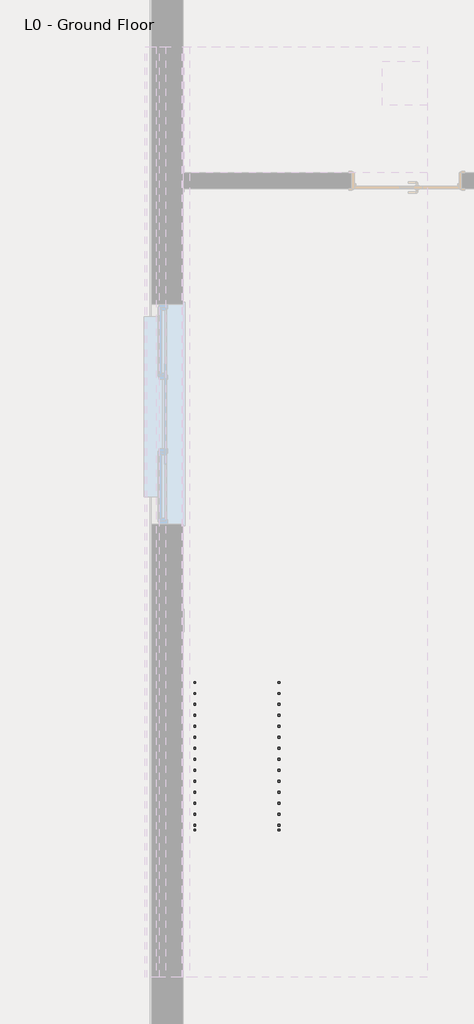
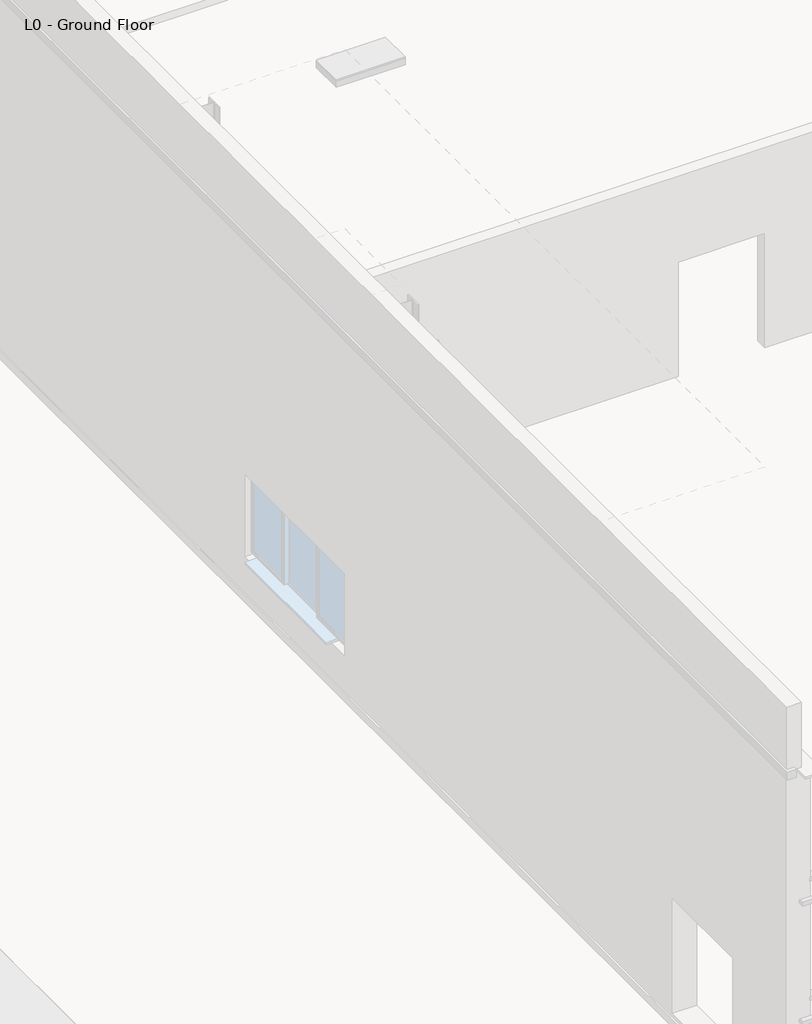
# One storey, part 8 of 14: 2 railings.
"""IFC4 building model written with IfcOpenShell, lengths in millimetres."""

import ifcopenshell
import ifcopenshell.guid

model = None  # the IFC model being written
_history = None  # IfcOwnerHistory: only IFC2X3 demands one
_inside = {}  # id of a spatial element -> (the spatial element, [elements in it])
_under = {}  # id of a project, library or spatial element -> (it, [spatial elements below it])
_declared = {}  # id of a project -> (the project, [libraries it declares])
_typed = {}  # id of a type object -> (the type object, [elements of that type])
_made_of = {}  # id of a material, layer set ... -> (it, [elements and type objects made of it])


def new_model(schema):
    """Start an empty IFC model of exactly this schema.

    Asked for "IFC4X3", IfcOpenShell would pick the latest addendum, in which some entities
    have other attributes; the version numbers below select the first issue.
    IFC2X3 requires an IfcOwnerHistory on every rooted entity: one is made here for all.
    """
    global model, _history
    if schema == "IFC4X3":
        model = ifcopenshell.file(schema_version=(4, 3, 0, 0))
    else:
        model = ifcopenshell.file(schema=schema)
    _inside.clear()
    _under.clear()
    _declared.clear()
    _typed.clear()
    _made_of.clear()
    _history = None
    if model.schema == "IFC2X3":
        org = make("IfcOrganization", Name="unknown")
        user = make(
            "IfcPersonAndOrganization",
            ThePerson=make("IfcPerson", FamilyName="unknown"),
            TheOrganization=org,
        )
        app = make(
            "IfcApplication",
            ApplicationDeveloper=org,
            Version="unknown",
            ApplicationFullName="unknown",
            ApplicationIdentifier="unknown",
        )
        _history = make(
            "IfcOwnerHistory",
            OwningUser=user,
            OwningApplication=app,
            ChangeAction="ADDED",
            CreationDate=0,
        )
    return model


def make(cls, **values):
    """One entity of the class cls with the attributes given. An attribute that is None is left unset."""
    return model.create_entity(
        cls, **{name: value for name, value in values.items() if value is not None}
    )


def rooted(cls, **values):
    """An entity with a GlobalId (a new one), such as an element, a storey or a relation."""
    return make(cls, GlobalId=ifcopenshell.guid.new(), OwnerHistory=_history, **values)


def si_unit(unit_type, name, prefix=None):
    """IfcSIUnit, for example si_unit("LENGTHUNIT", "METRE", prefix="MILLI")."""
    return make("IfcSIUnit", UnitType=unit_type, Prefix=prefix, Name=name)


def assignment(units):
    """IfcUnitAssignment: the units of a project."""
    return None if units is None else make("IfcUnitAssignment", Units=units)


def point(xyz):
    """IfcCartesianPoint."""
    return None if xyz is None else make("IfcCartesianPoint", Coordinates=xyz)


def direction(xyz):
    """IfcDirection."""
    return None if xyz is None else make("IfcDirection", DirectionRatios=xyz)


def frame(location, z_axis=None, x_axis=None):
    """IfcAxis2Placement3D, a coordinate frame: its origin and axes. An axis left out is left unset."""
    return make(
        "IfcAxis2Placement3D",
        Location=point(location),
        Axis=direction(z_axis),
        RefDirection=direction(x_axis),
    )


def origin():
    """The frame at (0, 0, 0) with its axes left unset."""
    return frame((0.0, 0.0, 0.0))


def place(relative_to, where):
    """IfcLocalPlacement: puts the frame where relative to a parent placement (None: the world)."""
    return make(
        "IfcLocalPlacement", PlacementRelTo=relative_to, RelativePlacement=where
    )


def context(
    kind, dimensions, precision=None, world=None, true_north=None, identifier=None
):
    """IfcGeometricRepresentationContext, for example the 3D "Model" context."""
    return make(
        "IfcGeometricRepresentationContext",
        ContextIdentifier=identifier,
        ContextType=kind,
        CoordinateSpaceDimension=dimensions,
        Precision=precision,
        WorldCoordinateSystem=world,
        TrueNorth=true_north,
    )


def project(units=None, contexts=None):
    """IfcProject with its units and contexts."""
    return rooted(
        "IfcProject",
        Name="project",
        RepresentationContexts=contexts,
        UnitsInContext=assignment(units),
    )


def spatial(cls, under=None, at=None, **own):
    """A site, building, storey or space (cls), placed at a placement, below another one or the project."""
    s = rooted(cls, ObjectPlacement=at, **own)
    if under is not None:
        _under.setdefault(under.id(), (under, []))[1].append(s)
    return s


def polyline(points):
    """IfcPolyline through the points."""
    return make("IfcPolyline", Points=[point(p) for p in points])


def outline(outer, holes=None, kind="AREA"):
    """IfcArbitraryClosedProfileDef: a profile drawn as a closed curve; with holes, ...WithVoids."""
    if holes is None:
        return make("IfcArbitraryClosedProfileDef", ProfileType=kind, OuterCurve=outer)
    return make(
        "IfcArbitraryProfileDefWithVoids",
        ProfileType=kind,
        OuterCurve=outer,
        InnerCurves=holes,
    )


def extrude(swept, where, along, depth):
    """IfcExtrudedAreaSolid: the profile swept, set in the frame where, extruded along a direction by depth."""
    return make(
        "IfcExtrudedAreaSolid",
        SweptArea=swept,
        Position=where,
        ExtrudedDirection=direction(along),
        Depth=depth,
    )


def faces_of(points, faces, orient=None, outer=None):
    """IfcFace entities. A face is a list of loops; a loop is a list of indices into points, from 0.

    orient and outer hold one flag for each loop. By default every Orientation is true, the
    first loop of a face is its IfcFaceOuterBound and the others are IfcFaceBound.
    """
    made = []
    for i, loops in enumerate(faces):
        bounds = []
        for j, loop in enumerate(loops):
            is_outer = j == 0 if outer is None else outer[i][j]
            bounds.append(
                make(
                    "IfcFaceOuterBound" if is_outer else "IfcFaceBound",
                    Bound=make("IfcPolyLoop", Polygon=[points[k] for k in loop]),
                    Orientation=True if orient is None else orient[i][j],
                )
            )
        made.append(make("IfcFace", Bounds=bounds))
    return made


def faceted_brep(points, faces, orient=None, outer=None, voids=None):
    """IfcFacetedBrep: a solid bounded by flat faces; with voids (closed shells), ...WithVoids."""
    shared = [point(p) for p in points]
    hull = make("IfcClosedShell", CfsFaces=faces_of(shared, faces, orient, outer))
    if voids is None:
        return make("IfcFacetedBrep", Outer=hull)
    return make(
        "IfcFacetedBrepWithVoids",
        Outer=hull,
        Voids=[
            make(cls, CfsFaces=faces_of(shared, fs, o, b)) for cls, fs, o, b in voids
        ],
    )


def shape(context_of_items, identifier, shape_type, items):
    """IfcShapeRepresentation: the items that make up one representation, for example the "Body"."""
    return make(
        "IfcShapeRepresentation",
        ContextOfItems=context_of_items,
        RepresentationIdentifier=identifier,
        RepresentationType=shape_type,
        Items=items,
    )


def made_of(thing, what):
    """Note that an element or type object is made of a material, layer set ...; save() writes the relation."""
    if what is not None:
        _made_of.setdefault(what.id(), (what, []))[1].append(thing)
    return thing


def element(
    cls,
    number,
    at=None,
    inside=None,
    cuts=None,
    type_object=None,
    material=None,
    context=None,
    identifier="Body",
    shape_type=None,
    held_by="IfcProductDefinitionShape",
    body=None,
    shapes=None,
    **own,
):
    """One element of the class cls, such as IfcWall. Its Tag is "e" and its number.

    at: its placement. inside: the storey or other place that contains it. cuts: it is an
    opening in that element (IfcRelVoidsElement). A single representation is given by context,
    identifier, shape_type and body (its items); several are given by shapes. held_by: the class
    of the entity that holds the representations. save() writes the other relations.
    """
    e = rooted(cls, Tag="e%d" % number, ObjectPlacement=at, **own)
    if body is not None:
        shapes = [shape(context, identifier, shape_type, body)]
    if shapes is not None:
        e.Representation = make(held_by, Representations=shapes)
    if inside is not None:
        _inside.setdefault(inside.id(), (inside, []))[1].append(e)
    if cuts is not None:
        rooted(
            "IfcRelVoidsElement", RelatingBuildingElement=cuts, RelatedOpeningElement=e
        )
    if type_object is not None:
        _typed.setdefault(type_object.id(), (type_object, []))[1].append(e)
    return made_of(e, material)


def aggregate(whole, parts):
    """IfcRelAggregates: a whole, such as a stair, and the parts it consists of."""
    return rooted("IfcRelAggregates", RelatingObject=whole, RelatedObjects=parts)


def save(model, path):
    """Write the relations noted so far, then the file.

    IfcRelAggregates (storeys below a building ...), IfcRelContainedInSpatialStructure (elements
    in a storey), IfcRelDefinesByType, IfcRelAssociatesMaterial and IfcRelDeclares: one each for
    every whole, place, type object, material and project.
    """
    for whole, parts in _under.values():
        aggregate(whole, parts)
    for where, things in _inside.values():
        rooted(
            "IfcRelContainedInSpatialStructure",
            RelatedElements=things,
            RelatingStructure=where,
        )
    for kind, things in _typed.values():
        rooted("IfcRelDefinesByType", RelatedObjects=things, RelatingType=kind)
    for what, things in _made_of.values():
        rooted("IfcRelAssociatesMaterial", RelatedObjects=things, RelatingMaterial=what)
    for by, libraries in _declared.values():
        rooted("IfcRelDeclares", RelatingContext=by, RelatedDefinitions=libraries)
    model.write(path)


model = new_model("IFC4")

# Units and contexts
model_context = context("Model", 3, world=origin())
ifc_project = project(units=[si_unit("LENGTHUNIT", "METRE", prefix="MILLI")], contexts=[model_context])

# Site, building, storey
site = spatial("IfcSite", under=ifc_project)
building = spatial("IfcBuilding", under=site)
storey = spatial("IfcBuildingStorey", under=building, Name="L0 - Ground Floor", Elevation=0.0)

# Railings
placement = place(None, origin())
element("IfcRailing", 1, ObjectType="1100mm", at=placement, inside=storey, context=model_context, shape_type="SolidModel", body=[
    faceted_brep([(-5716.2916692, -13929.5546689, 1266.6666667), (-5716.2916692, -13929.5546689, 1209.4687214), (-5666.2916692, -13929.5546689, 1209.4687214), (-5666.2916692, -13929.5546689, 1266.6666667), (-5716.2916692, -11829.5546689, 2433.3333333), (-5716.2916692, -11816.5983675, 2383.3333333), (-5666.2916692, -11816.5983675, 2383.3333333), (-5666.2916692, -11829.5546689, 2433.3333333), (-5716.2916692, -10929.5546689, 2433.3333333), (-5716.2916692, -10916.5983675, 2383.3333333), (-5666.2916692, -10916.5983675, 2383.3333333), (-5666.2916692, -10929.5546689, 2433.3333333), (-5716.2916692, -8529.5546689, 3766.6666667), (-5716.2916692, -8516.5983675, 3716.6666667), (-5666.2916692, -8516.5983675, 3716.6666667), (-5666.2916692, -8529.5546689, 3766.6666667), (-5716.2916692, -7629.5546689, 3766.6666667), (-5716.2916692, -7616.5983675, 3716.6666667), (-5666.2916692, -7616.5983675, 3716.6666667), (-5666.2916692, -7629.5546689, 3766.6666667), (-5716.2916692, -5229.5546689, 5100.0), (-5666.2916692, -5229.5546689, 5100.0), (-5666.2916692, -5229.5546689, 5042.8020548), (-5716.2916692, -5229.5546689, 5042.8020548)], [[[0, 1, 2, 3]], [[1, 0, 4, 5]], [[2, 1, 5, 6]], [[3, 2, 6, 7]], [[0, 3, 7, 4]], [[5, 4, 8, 9]], [[6, 5, 9, 10]], [[7, 6, 10, 11]], [[4, 7, 11, 8]], [[9, 8, 12, 13]], [[10, 9, 13, 14]], [[11, 10, 14, 15]], [[8, 11, 15, 12]], [[13, 12, 16, 17]], [[14, 13, 17, 18]], [[15, 14, 18, 19]], [[12, 15, 19, 16]], [[20, 21, 22, 23]], [[17, 16, 20, 23]], [[18, 17, 23, 22]], [[19, 18, 22, 21]], [[16, 19, 21, 20]]]),
    extrude(outline(polyline([(-5317.0546689, 3833.3333333), (-5317.0546689, 4994.1909437), (-5292.0546689, 5008.0798326), (-5292.0546689, 3833.3333333), (-5317.0546689, 3833.3333333)])), frame((-5703.7916692, 0.0, 0.0), z_axis=(1.0, 0.0, 0.0), x_axis=(0.0, 1.0, 0.0)), (0.0, 0.0, 1.0), 25.0),
    extrude(outline(polyline([(-5467.0546689, 3833.3333333), (-5467.0546689, 4910.8576103), (-5442.0546689, 4924.7464992), (-5442.0546689, 3833.3333333), (-5467.0546689, 3833.3333333)])), frame((-5703.7916692, 0.0, 0.0), z_axis=(1.0, 0.0, 0.0), x_axis=(0.0, 1.0, 0.0)), (0.0, 0.0, 1.0), 25.0),
    extrude(outline(polyline([(-5617.0546689, 3666.6666667), (-5617.0546689, 4827.524277), (-5592.0546689, 4841.4131659), (-5592.0546689, 3666.6666667), (-5617.0546689, 3666.6666667)])), frame((-5703.7916692, 0.0, 0.0), z_axis=(1.0, 0.0, 0.0), x_axis=(0.0, 1.0, 0.0)), (0.0, 0.0, 1.0), 25.0),
    extrude(outline(polyline([(-5767.0546689, 3666.6666667), (-5767.0546689, 4744.1909437), (-5742.0546689, 4758.0798326), (-5742.0546689, 3666.6666667), (-5767.0546689, 3666.6666667)])), frame((-5703.7916692, 0.0, 0.0), z_axis=(1.0, 0.0, 0.0), x_axis=(0.0, 1.0, 0.0)), (0.0, 0.0, 1.0), 25.0),
    extrude(outline(polyline([(-5917.0546689, 3500.0), (-5917.0546689, 4660.8576103), (-5892.0546689, 4674.7464992), (-5892.0546689, 3500.0), (-5917.0546689, 3500.0)])), frame((-5703.7916692, 0.0, 0.0), z_axis=(1.0, 0.0, 0.0), x_axis=(0.0, 1.0, 0.0)), (0.0, 0.0, 1.0), 25.0),
    extrude(outline(polyline([(-6067.0546689, 3500.0), (-6067.0546689, 4577.524277), (-6042.0546689, 4591.4131659), (-6042.0546689, 3500.0), (-6067.0546689, 3500.0)])), frame((-5703.7916692, 0.0, 0.0), z_axis=(1.0, 0.0, 0.0), x_axis=(0.0, 1.0, 0.0)), (0.0, 0.0, 1.0), 25.0),
    extrude(outline(polyline([(-6217.0546689, 3333.3333333), (-6217.0546689, 4494.1909437), (-6192.0546689, 4508.0798326), (-6192.0546689, 3333.3333333), (-6217.0546689, 3333.3333333)])), frame((-5703.7916692, 0.0, 0.0), z_axis=(1.0, 0.0, 0.0), x_axis=(0.0, 1.0, 0.0)), (0.0, 0.0, 1.0), 25.0),
    extrude(outline(polyline([(-6367.0546689, 3333.3333333), (-6367.0546689, 4410.8576103), (-6342.0546689, 4424.7464992), (-6342.0546689, 3333.3333333), (-6367.0546689, 3333.3333333)])), frame((-5703.7916692, 0.0, 0.0), z_axis=(1.0, 0.0, 0.0), x_axis=(0.0, 1.0, 0.0)), (0.0, 0.0, 1.0), 25.0),
    extrude(outline(polyline([(-6517.0546689, 3166.6666667), (-6517.0546689, 4327.524277), (-6492.0546689, 4341.4131659), (-6492.0546689, 3166.6666667), (-6517.0546689, 3166.6666667)])), frame((-5703.7916692, 0.0, 0.0), z_axis=(1.0, 0.0, 0.0), x_axis=(0.0, 1.0, 0.0)), (0.0, 0.0, 1.0), 25.0),
    extrude(outline(polyline([(-6667.0546689, 3166.6666667), (-6667.0546689, 4244.1909437), (-6642.0546689, 4258.0798326), (-6642.0546689, 3166.6666667), (-6667.0546689, 3166.6666667)])), frame((-5703.7916692, 0.0, 0.0), z_axis=(1.0, 0.0, 0.0), x_axis=(0.0, 1.0, 0.0)), (0.0, 0.0, 1.0), 25.0),
    extrude(outline(polyline([(-6817.0546689, 3000.0), (-6817.0546689, 4160.8576103), (-6792.0546689, 4174.7464992), (-6792.0546689, 3000.0), (-6817.0546689, 3000.0)])), frame((-5703.7916692, 0.0, 0.0), z_axis=(1.0, 0.0, 0.0), x_axis=(0.0, 1.0, 0.0)), (0.0, 0.0, 1.0), 25.0),
    extrude(outline(polyline([(-6967.0546689, 3000.0), (-6967.0546689, 4077.524277), (-6942.0546689, 4091.4131659), (-6942.0546689, 3000.0), (-6967.0546689, 3000.0)])), frame((-5703.7916692, 0.0, 0.0), z_axis=(1.0, 0.0, 0.0), x_axis=(0.0, 1.0, 0.0)), (0.0, 0.0, 1.0), 25.0),
    extrude(outline(polyline([(-7117.0546689, 2833.3333333), (-7117.0546689, 3994.1909437), (-7092.0546689, 4008.0798326), (-7092.0546689, 2833.3333333), (-7117.0546689, 2833.3333333)])), frame((-5703.7916692, 0.0, 0.0), z_axis=(1.0, 0.0, 0.0), x_axis=(0.0, 1.0, 0.0)), (0.0, 0.0, 1.0), 25.0),
    extrude(outline(polyline([(-7267.0546689, 2833.3333333), (-7267.0546689, 3910.8576103), (-7242.0546689, 3924.7464992), (-7242.0546689, 2833.3333333), (-7267.0546689, 2833.3333333)])), frame((-5703.7916692, 0.0, 0.0), z_axis=(1.0, 0.0, 0.0), x_axis=(0.0, 1.0, 0.0)), (0.0, 0.0, 1.0), 25.0),
    extrude(outline(polyline([(-7417.0546689, 2666.6666667), (-7417.0546689, 3827.524277), (-7392.0546689, 3841.4131659), (-7392.0546689, 2666.6666667), (-7417.0546689, 2666.6666667)])), frame((-5703.7916692, 0.0, 0.0), z_axis=(1.0, 0.0, 0.0), x_axis=(0.0, 1.0, 0.0)), (0.0, 0.0, 1.0), 25.0),
    extrude(outline(polyline([(-7567.0546689, 2666.6666667), (-7567.0546689, 3744.1909437), (-7542.0546689, 3758.0798326), (-7542.0546689, 2666.6666667), (-7567.0546689, 2666.6666667)])), frame((-5703.7916692, 0.0, 0.0), z_axis=(1.0, 0.0, 0.0), x_axis=(0.0, 1.0, 0.0)), (0.0, 0.0, 1.0), 25.0),
    extrude(outline(polyline([(-5678.7916692, -7717.0546689), (-5703.7916692, -7717.0546689), (-5703.7916692, -7692.0546689), (-5678.7916692, -7692.0546689), (-5678.7916692, -7717.0546689)])), frame((0.0, 0.0, 2666.6666667), z_axis=(0.0, 0.0, 1.0), x_axis=(1.0, 0.0, 0.0)), (0.0, 0.0, 1.0), 1050.0),
    extrude(outline(polyline([(-5678.7916692, -7867.0546689), (-5703.7916692, -7867.0546689), (-5703.7916692, -7842.0546689), (-5678.7916692, -7842.0546689), (-5678.7916692, -7867.0546689)])), frame((0.0, 0.0, 2666.6666667), z_axis=(0.0, 0.0, 1.0), x_axis=(1.0, 0.0, 0.0)), (0.0, 0.0, 1.0), 1050.0),
    extrude(outline(polyline([(-5678.7916692, -8017.0546689), (-5703.7916692, -8017.0546689), (-5703.7916692, -7992.0546689), (-5678.7916692, -7992.0546689), (-5678.7916692, -8017.0546689)])), frame((0.0, 0.0, 2666.6666667), z_axis=(0.0, 0.0, 1.0), x_axis=(1.0, 0.0, 0.0)), (0.0, 0.0, 1.0), 1050.0),
    extrude(outline(polyline([(-5678.7916692, -8167.0546689), (-5703.7916692, -8167.0546689), (-5703.7916692, -8142.0546689), (-5678.7916692, -8142.0546689), (-5678.7916692, -8167.0546689)])), frame((0.0, 0.0, 2666.6666667), z_axis=(0.0, 0.0, 1.0), x_axis=(1.0, 0.0, 0.0)), (0.0, 0.0, 1.0), 1050.0),
    extrude(outline(polyline([(-5678.7916692, -8317.0546689), (-5703.7916692, -8317.0546689), (-5703.7916692, -8292.0546689), (-5678.7916692, -8292.0546689), (-5678.7916692, -8317.0546689)])), frame((0.0, 0.0, 2666.6666667), z_axis=(0.0, 0.0, 1.0), x_axis=(1.0, 0.0, 0.0)), (0.0, 0.0, 1.0), 1050.0),
    extrude(outline(polyline([(-5678.7916692, -8467.0546689), (-5703.7916692, -8467.0546689), (-5703.7916692, -8442.0546689), (-5678.7916692, -8442.0546689), (-5678.7916692, -8467.0546689)])), frame((0.0, 0.0, 2666.6666667), z_axis=(0.0, 0.0, 1.0), x_axis=(1.0, 0.0, 0.0)), (0.0, 0.0, 1.0), 1050.0),
    extrude(outline(polyline([(-8617.0546689, 2500.0), (-8617.0546689, 3660.8576103), (-8592.0546689, 3674.7464992), (-8592.0546689, 2500.0), (-8617.0546689, 2500.0)])), frame((-5703.7916692, 0.0, 0.0), z_axis=(1.0, 0.0, 0.0), x_axis=(0.0, 1.0, 0.0)), (0.0, 0.0, 1.0), 25.0),
    extrude(outline(polyline([(-8767.0546689, 2500.0), (-8767.0546689, 3577.524277), (-8742.0546689, 3591.4131659), (-8742.0546689, 2500.0), (-8767.0546689, 2500.0)])), frame((-5703.7916692, 0.0, 0.0), z_axis=(1.0, 0.0, 0.0), x_axis=(0.0, 1.0, 0.0)), (0.0, 0.0, 1.0), 25.0),
    extrude(outline(polyline([(-8917.0546689, 2333.3333333), (-8917.0546689, 3494.1909437), (-8892.0546689, 3508.0798326), (-8892.0546689, 2333.3333333), (-8917.0546689, 2333.3333333)])), frame((-5703.7916692, 0.0, 0.0), z_axis=(1.0, 0.0, 0.0), x_axis=(0.0, 1.0, 0.0)), (0.0, 0.0, 1.0), 25.0),
    extrude(outline(polyline([(-9067.0546689, 2333.3333333), (-9067.0546689, 3410.8576103), (-9042.0546689, 3424.7464992), (-9042.0546689, 2333.3333333), (-9067.0546689, 2333.3333333)])), frame((-5703.7916692, 0.0, 0.0), z_axis=(1.0, 0.0, 0.0), x_axis=(0.0, 1.0, 0.0)), (0.0, 0.0, 1.0), 25.0),
    extrude(outline(polyline([(-9217.0546689, 2166.6666667), (-9217.0546689, 3327.524277), (-9192.0546689, 3341.4131659), (-9192.0546689, 2166.6666667), (-9217.0546689, 2166.6666667)])), frame((-5703.7916692, 0.0, 0.0), z_axis=(1.0, 0.0, 0.0), x_axis=(0.0, 1.0, 0.0)), (0.0, 0.0, 1.0), 25.0),
    extrude(outline(polyline([(-9367.0546689, 2166.6666667), (-9367.0546689, 3244.1909437), (-9342.0546689, 3258.0798326), (-9342.0546689, 2166.6666667), (-9367.0546689, 2166.6666667)])), frame((-5703.7916692, 0.0, 0.0), z_axis=(1.0, 0.0, 0.0), x_axis=(0.0, 1.0, 0.0)), (0.0, 0.0, 1.0), 25.0),
    extrude(outline(polyline([(-9517.0546689, 2000.0), (-9517.0546689, 3160.8576103), (-9492.0546689, 3174.7464992), (-9492.0546689, 2000.0), (-9517.0546689, 2000.0)])), frame((-5703.7916692, 0.0, 0.0), z_axis=(1.0, 0.0, 0.0), x_axis=(0.0, 1.0, 0.0)), (0.0, 0.0, 1.0), 25.0),
    extrude(outline(polyline([(-9667.0546689, 2000.0), (-9667.0546689, 3077.524277), (-9642.0546689, 3091.4131659), (-9642.0546689, 2000.0), (-9667.0546689, 2000.0)])), frame((-5703.7916692, 0.0, 0.0), z_axis=(1.0, 0.0, 0.0), x_axis=(0.0, 1.0, 0.0)), (0.0, 0.0, 1.0), 25.0),
    extrude(outline(polyline([(-9817.0546689, 1833.3333333), (-9817.0546689, 2994.1909437), (-9792.0546689, 3008.0798326), (-9792.0546689, 1833.3333333), (-9817.0546689, 1833.3333333)])), frame((-5703.7916692, 0.0, 0.0), z_axis=(1.0, 0.0, 0.0), x_axis=(0.0, 1.0, 0.0)), (0.0, 0.0, 1.0), 25.0),
    extrude(outline(polyline([(-9967.0546689, 1833.3333333), (-9967.0546689, 2910.8576103), (-9942.0546689, 2924.7464992), (-9942.0546689, 1833.3333333), (-9967.0546689, 1833.3333333)])), frame((-5703.7916692, 0.0, 0.0), z_axis=(1.0, 0.0, 0.0), x_axis=(0.0, 1.0, 0.0)), (0.0, 0.0, 1.0), 25.0),
    extrude(outline(polyline([(-10117.0546689, 1666.6666667), (-10117.0546689, 2827.524277), (-10092.0546689, 2841.4131659), (-10092.0546689, 1666.6666667), (-10117.0546689, 1666.6666667)])), frame((-5703.7916692, 0.0, 0.0), z_axis=(1.0, 0.0, 0.0), x_axis=(0.0, 1.0, 0.0)), (0.0, 0.0, 1.0), 25.0),
    extrude(outline(polyline([(-10267.0546689, 1666.6666667), (-10267.0546689, 2744.1909437), (-10242.0546689, 2758.0798326), (-10242.0546689, 1666.6666667), (-10267.0546689, 1666.6666667)])), frame((-5703.7916692, 0.0, 0.0), z_axis=(1.0, 0.0, 0.0), x_axis=(0.0, 1.0, 0.0)), (0.0, 0.0, 1.0), 25.0),
    extrude(outline(polyline([(-10417.0546689, 1500.0), (-10417.0546689, 2660.8576103), (-10392.0546689, 2674.7464992), (-10392.0546689, 1500.0), (-10417.0546689, 1500.0)])), frame((-5703.7916692, 0.0, 0.0), z_axis=(1.0, 0.0, 0.0), x_axis=(0.0, 1.0, 0.0)), (0.0, 0.0, 1.0), 25.0),
    extrude(outline(polyline([(-10567.0546689, 1500.0), (-10567.0546689, 2577.524277), (-10542.0546689, 2591.4131659), (-10542.0546689, 1500.0), (-10567.0546689, 1500.0)])), frame((-5703.7916692, 0.0, 0.0), z_axis=(1.0, 0.0, 0.0), x_axis=(0.0, 1.0, 0.0)), (0.0, 0.0, 1.0), 25.0),
    extrude(outline(polyline([(-10717.0546689, 1333.3333333), (-10717.0546689, 2494.1909437), (-10692.0546689, 2508.0798326), (-10692.0546689, 1333.3333333), (-10717.0546689, 1333.3333333)])), frame((-5703.7916692, 0.0, 0.0), z_axis=(1.0, 0.0, 0.0), x_axis=(0.0, 1.0, 0.0)), (0.0, 0.0, 1.0), 25.0),
    extrude(outline(polyline([(-10867.0546689, 1333.3333333), (-10867.0546689, 2410.8576103), (-10842.0546689, 2424.7464992), (-10842.0546689, 1333.3333333), (-10867.0546689, 1333.3333333)])), frame((-5703.7916692, 0.0, 0.0), z_axis=(1.0, 0.0, 0.0), x_axis=(0.0, 1.0, 0.0)), (0.0, 0.0, 1.0), 25.0),
    extrude(outline(polyline([(-5678.7916692, -11017.0546689), (-5703.7916692, -11017.0546689), (-5703.7916692, -10992.0546689), (-5678.7916692, -10992.0546689), (-5678.7916692, -11017.0546689)])), frame((0.0, 0.0, 1333.3333333), z_axis=(0.0, 0.0, 1.0), x_axis=(1.0, 0.0, 0.0)), (0.0, 0.0, 1.0), 1050.0),
    extrude(outline(polyline([(-5678.7916692, -11167.0546689), (-5703.7916692, -11167.0546689), (-5703.7916692, -11142.0546689), (-5678.7916692, -11142.0546689), (-5678.7916692, -11167.0546689)])), frame((0.0, 0.0, 1333.3333333), z_axis=(0.0, 0.0, 1.0), x_axis=(1.0, 0.0, 0.0)), (0.0, 0.0, 1.0), 1050.0),
    extrude(outline(polyline([(-5678.7916692, -11317.0546689), (-5703.7916692, -11317.0546689), (-5703.7916692, -11292.0546689), (-5678.7916692, -11292.0546689), (-5678.7916692, -11317.0546689)])), frame((0.0, 0.0, 1333.3333333), z_axis=(0.0, 0.0, 1.0), x_axis=(1.0, 0.0, 0.0)), (0.0, 0.0, 1.0), 1050.0),
    extrude(outline(polyline([(-5678.7916692, -11467.0546689), (-5703.7916692, -11467.0546689), (-5703.7916692, -11442.0546689), (-5678.7916692, -11442.0546689), (-5678.7916692, -11467.0546689)])), frame((0.0, 0.0, 1333.3333333), z_axis=(0.0, 0.0, 1.0), x_axis=(1.0, 0.0, 0.0)), (0.0, 0.0, 1.0), 1050.0),
    extrude(outline(polyline([(-5678.7916692, -11617.0546689), (-5703.7916692, -11617.0546689), (-5703.7916692, -11592.0546689), (-5678.7916692, -11592.0546689), (-5678.7916692, -11617.0546689)])), frame((0.0, 0.0, 1333.3333333), z_axis=(0.0, 0.0, 1.0), x_axis=(1.0, 0.0, 0.0)), (0.0, 0.0, 1.0), 1050.0),
    extrude(outline(polyline([(-5678.7916692, -11767.0546689), (-5703.7916692, -11767.0546689), (-5703.7916692, -11742.0546689), (-5678.7916692, -11742.0546689), (-5678.7916692, -11767.0546689)])), frame((0.0, 0.0, 1333.3333333), z_axis=(0.0, 0.0, 1.0), x_axis=(1.0, 0.0, 0.0)), (0.0, 0.0, 1.0), 1050.0),
    extrude(outline(polyline([(-11917.0546689, 1166.6666667), (-11917.0546689, 2327.524277), (-11892.0546689, 2341.4131659), (-11892.0546689, 1166.6666667), (-11917.0546689, 1166.6666667)])), frame((-5703.7916692, 0.0, 0.0), z_axis=(1.0, 0.0, 0.0), x_axis=(0.0, 1.0, 0.0)), (0.0, 0.0, 1.0), 25.0),
    extrude(outline(polyline([(-12067.0546689, 1166.6666667), (-12067.0546689, 2244.1909437), (-12042.0546689, 2258.0798326), (-12042.0546689, 1166.6666667), (-12067.0546689, 1166.6666667)])), frame((-5703.7916692, 0.0, 0.0), z_axis=(1.0, 0.0, 0.0), x_axis=(0.0, 1.0, 0.0)), (0.0, 0.0, 1.0), 25.0),
    extrude(outline(polyline([(-12217.0546689, 1000.0), (-12217.0546689, 2160.8576103), (-12192.0546689, 2174.7464992), (-12192.0546689, 1000.0), (-12217.0546689, 1000.0)])), frame((-5703.7916692, 0.0, 0.0), z_axis=(1.0, 0.0, 0.0), x_axis=(0.0, 1.0, 0.0)), (0.0, 0.0, 1.0), 25.0),
    extrude(outline(polyline([(-12367.0546689, 1000.0), (-12367.0546689, 2077.524277), (-12342.0546689, 2091.4131659), (-12342.0546689, 1000.0), (-12367.0546689, 1000.0)])), frame((-5703.7916692, 0.0, 0.0), z_axis=(1.0, 0.0, 0.0), x_axis=(0.0, 1.0, 0.0)), (0.0, 0.0, 1.0), 25.0),
    extrude(outline(polyline([(-12517.0546689, 833.3333333), (-12517.0546689, 1994.1909437), (-12492.0546689, 2008.0798326), (-12492.0546689, 833.3333333), (-12517.0546689, 833.3333333)])), frame((-5703.7916692, 0.0, 0.0), z_axis=(1.0, 0.0, 0.0), x_axis=(0.0, 1.0, 0.0)), (0.0, 0.0, 1.0), 25.0),
    extrude(outline(polyline([(-12667.0546689, 833.3333333), (-12667.0546689, 1910.8576103), (-12642.0546689, 1924.7464992), (-12642.0546689, 833.3333333), (-12667.0546689, 833.3333333)])), frame((-5703.7916692, 0.0, 0.0), z_axis=(1.0, 0.0, 0.0), x_axis=(0.0, 1.0, 0.0)), (0.0, 0.0, 1.0), 25.0),
    extrude(outline(polyline([(-12817.0546689, 666.6666667), (-12817.0546689, 1827.524277), (-12792.0546689, 1841.4131659), (-12792.0546689, 666.6666667), (-12817.0546689, 666.6666667)])), frame((-5703.7916692, 0.0, 0.0), z_axis=(1.0, 0.0, 0.0), x_axis=(0.0, 1.0, 0.0)), (0.0, 0.0, 1.0), 25.0),
    extrude(outline(polyline([(-12967.0546689, 666.6666667), (-12967.0546689, 1744.1909437), (-12942.0546689, 1758.0798326), (-12942.0546689, 666.6666667), (-12967.0546689, 666.6666667)])), frame((-5703.7916692, 0.0, 0.0), z_axis=(1.0, 0.0, 0.0), x_axis=(0.0, 1.0, 0.0)), (0.0, 0.0, 1.0), 25.0),
    extrude(outline(polyline([(-13117.0546689, 500.0), (-13117.0546689, 1660.8576103), (-13092.0546689, 1674.7464992), (-13092.0546689, 500.0), (-13117.0546689, 500.0)])), frame((-5703.7916692, 0.0, 0.0), z_axis=(1.0, 0.0, 0.0), x_axis=(0.0, 1.0, 0.0)), (0.0, 0.0, 1.0), 25.0),
    extrude(outline(polyline([(-13267.0546689, 500.0), (-13267.0546689, 1577.524277), (-13242.0546689, 1591.4131659), (-13242.0546689, 500.0), (-13267.0546689, 500.0)])), frame((-5703.7916692, 0.0, 0.0), z_axis=(1.0, 0.0, 0.0), x_axis=(0.0, 1.0, 0.0)), (0.0, 0.0, 1.0), 25.0),
    extrude(outline(polyline([(-13417.0546689, 333.3333333), (-13417.0546689, 1494.1909437), (-13392.0546689, 1508.0798326), (-13392.0546689, 333.3333333), (-13417.0546689, 333.3333333)])), frame((-5703.7916692, 0.0, 0.0), z_axis=(1.0, 0.0, 0.0), x_axis=(0.0, 1.0, 0.0)), (0.0, 0.0, 1.0), 25.0),
    extrude(outline(polyline([(-13567.0546689, 333.3333333), (-13567.0546689, 1410.8576103), (-13542.0546689, 1424.7464992), (-13542.0546689, 333.3333333), (-13567.0546689, 333.3333333)])), frame((-5703.7916692, 0.0, 0.0), z_axis=(1.0, 0.0, 0.0), x_axis=(0.0, 1.0, 0.0)), (0.0, 0.0, 1.0), 25.0),
    extrude(outline(polyline([(-13717.0546689, 166.6666667), (-13717.0546689, 1327.524277), (-13692.0546689, 1341.4131659), (-13692.0546689, 166.6666667), (-13717.0546689, 166.6666667)])), frame((-5703.7916692, 0.0, 0.0), z_axis=(1.0, 0.0, 0.0), x_axis=(0.0, 1.0, 0.0)), (0.0, 0.0, 1.0), 25.0),
    extrude(outline(polyline([(-13867.0546689, 166.6666667), (-13867.0546689, 1244.1909437), (-13842.0546689, 1258.0798326), (-13842.0546689, 166.6666667), (-13867.0546689, 166.6666667)])), frame((-5703.7916692, 0.0, 0.0), z_axis=(1.0, 0.0, 0.0), x_axis=(0.0, 1.0, 0.0)), (0.0, 0.0, 1.0), 25.0),
    extrude(outline(polyline([(-5678.7916692, -7642.0546689), (-5703.7916692, -7642.0546689), (-5703.7916692, -7617.0546689), (-5678.7916692, -7617.0546689), (-5678.7916692, -7642.0546689)])), frame((0.0, 0.0, 2666.6666667), z_axis=(0.0, 0.0, 1.0), x_axis=(1.0, 0.0, 0.0)), (0.0, 0.0, 1.0), 1050.0),
    extrude(outline(polyline([(-8542.0546689, 2666.6666667), (-8542.0546689, 3702.524277), (-8517.0546689, 3716.4131659), (-8517.0546689, 2666.6666667), (-8542.0546689, 2666.6666667)])), frame((-5703.7916692, 0.0, 0.0), z_axis=(1.0, 0.0, 0.0), x_axis=(0.0, 1.0, 0.0)), (0.0, 0.0, 1.0), 25.0),
    extrude(outline(polyline([(-5678.7916692, -10942.0546689), (-5703.7916692, -10942.0546689), (-5703.7916692, -10917.0546689), (-5678.7916692, -10917.0546689), (-5678.7916692, -10942.0546689)])), frame((0.0, 0.0, 1333.3333333), z_axis=(0.0, 0.0, 1.0), x_axis=(1.0, 0.0, 0.0)), (0.0, 0.0, 1.0), 1050.0),
    extrude(outline(polyline([(-11842.0546689, 1333.3333333), (-11842.0546689, 2369.1909437), (-11817.0546689, 2383.0798326), (-11817.0546689, 1333.3333333), (-11842.0546689, 1333.3333333)])), frame((-5703.7916692, 0.0, 0.0), z_axis=(1.0, 0.0, 0.0), x_axis=(0.0, 1.0, 0.0)), (0.0, 0.0, 1.0), 25.0),
    extrude(outline(polyline([(-5254.5546689, 3833.3333333), (-5254.5546689, 5028.9131659), (-5229.5546689, 5042.8020548), (-5229.5546689, 3833.3333333), (-5254.5546689, 3833.3333333)])), frame((-5703.7916692, 0.0, 0.0), z_axis=(1.0, 0.0, 0.0), x_axis=(0.0, 1.0, 0.0)), (0.0, 0.0, 1.0), 25.0),
    extrude(outline(polyline([(-13929.5546689, 166.6666667), (-13929.5546689, 1209.4687214), (-13904.5546689, 1223.3576103), (-13904.5546689, 166.6666667), (-13929.5546689, 166.6666667)])), frame((-5703.7916692, 0.0, 0.0), z_axis=(1.0, 0.0, 0.0), x_axis=(0.0, 1.0, 0.0)), (0.0, 0.0, 1.0), 25.0),
])
element("IfcRailing", 2, ObjectType="1100mm", at=placement, inside=storey, context=model_context, shape_type="SolidModel", body=[
    faceted_brep([(-6865.4916692, -13929.5546689, 1266.6666667), (-6865.4916692, -13929.5546689, 1209.4687214), (-6815.4916692, -13929.5546689, 1209.4687214), (-6815.4916692, -13929.5546689, 1266.6666667), (-6865.4916692, -11829.5546689, 2433.3333333), (-6865.4916692, -11816.5983675, 2383.3333333), (-6815.4916692, -11816.5983675, 2383.3333333), (-6815.4916692, -11829.5546689, 2433.3333333), (-6865.4916692, -10929.5546689, 2433.3333333), (-6865.4916692, -10916.5983675, 2383.3333333), (-6815.4916692, -10916.5983675, 2383.3333333), (-6815.4916692, -10929.5546689, 2433.3333333), (-6865.4916692, -8529.5546689, 3766.6666667), (-6865.4916692, -8516.5983675, 3716.6666667), (-6815.4916692, -8516.5983675, 3716.6666667), (-6815.4916692, -8529.5546689, 3766.6666667), (-6865.4916692, -7629.5546689, 3766.6666667), (-6865.4916692, -7616.5983675, 3716.6666667), (-6815.4916692, -7616.5983675, 3716.6666667), (-6815.4916692, -7629.5546689, 3766.6666667), (-6865.4916692, -5229.5546689, 5100.0), (-6815.4916692, -5229.5546689, 5100.0), (-6815.4916692, -5229.5546689, 5042.8020548), (-6865.4916692, -5229.5546689, 5042.8020548)], [[[0, 1, 2, 3]], [[1, 0, 4, 5]], [[2, 1, 5, 6]], [[3, 2, 6, 7]], [[0, 3, 7, 4]], [[5, 4, 8, 9]], [[6, 5, 9, 10]], [[7, 6, 10, 11]], [[4, 7, 11, 8]], [[9, 8, 12, 13]], [[10, 9, 13, 14]], [[11, 10, 14, 15]], [[8, 11, 15, 12]], [[13, 12, 16, 17]], [[14, 13, 17, 18]], [[15, 14, 18, 19]], [[12, 15, 19, 16]], [[20, 21, 22, 23]], [[17, 16, 20, 23]], [[18, 17, 23, 22]], [[19, 18, 22, 21]], [[16, 19, 21, 20]]]),
    extrude(outline(polyline([(-5317.0546689, 4994.1909437), (-5292.0546689, 5008.0798326), (-5292.0546689, 3833.3333333), (-5317.0546689, 3833.3333333), (-5317.0546689, 4994.1909437)])), frame((-6852.9916692, 0.0, 0.0), z_axis=(1.0, 0.0, 0.0), x_axis=(0.0, 1.0, 0.0)), (0.0, 0.0, 1.0), 25.0),
    extrude(outline(polyline([(-5467.0546689, 4910.8576103), (-5442.0546689, 4924.7464992), (-5442.0546689, 3833.3333333), (-5467.0546689, 3833.3333333), (-5467.0546689, 4910.8576103)])), frame((-6852.9916692, 0.0, 0.0), z_axis=(1.0, 0.0, 0.0), x_axis=(0.0, 1.0, 0.0)), (0.0, 0.0, 1.0), 25.0),
    extrude(outline(polyline([(-5617.0546689, 4827.524277), (-5592.0546689, 4841.4131659), (-5592.0546689, 3666.6666667), (-5617.0546689, 3666.6666667), (-5617.0546689, 4827.524277)])), frame((-6852.9916692, 0.0, 0.0), z_axis=(1.0, 0.0, 0.0), x_axis=(0.0, 1.0, 0.0)), (0.0, 0.0, 1.0), 25.0),
    extrude(outline(polyline([(-5767.0546689, 4744.1909437), (-5742.0546689, 4758.0798326), (-5742.0546689, 3666.6666667), (-5767.0546689, 3666.6666667), (-5767.0546689, 4744.1909437)])), frame((-6852.9916692, 0.0, 0.0), z_axis=(1.0, 0.0, 0.0), x_axis=(0.0, 1.0, 0.0)), (0.0, 0.0, 1.0), 25.0),
    extrude(outline(polyline([(-5917.0546689, 4660.8576103), (-5892.0546689, 4674.7464992), (-5892.0546689, 3500.0), (-5917.0546689, 3500.0), (-5917.0546689, 4660.8576103)])), frame((-6852.9916692, 0.0, 0.0), z_axis=(1.0, 0.0, 0.0), x_axis=(0.0, 1.0, 0.0)), (0.0, 0.0, 1.0), 25.0),
    extrude(outline(polyline([(-6067.0546689, 4577.524277), (-6042.0546689, 4591.4131659), (-6042.0546689, 3500.0), (-6067.0546689, 3500.0), (-6067.0546689, 4577.524277)])), frame((-6852.9916692, 0.0, 0.0), z_axis=(1.0, 0.0, 0.0), x_axis=(0.0, 1.0, 0.0)), (0.0, 0.0, 1.0), 25.0),
    extrude(outline(polyline([(-6217.0546689, 4494.1909437), (-6192.0546689, 4508.0798326), (-6192.0546689, 3333.3333333), (-6217.0546689, 3333.3333333), (-6217.0546689, 4494.1909437)])), frame((-6852.9916692, 0.0, 0.0), z_axis=(1.0, 0.0, 0.0), x_axis=(0.0, 1.0, 0.0)), (0.0, 0.0, 1.0), 25.0),
    extrude(outline(polyline([(-6367.0546689, 4410.8576103), (-6342.0546689, 4424.7464992), (-6342.0546689, 3333.3333333), (-6367.0546689, 3333.3333333), (-6367.0546689, 4410.8576103)])), frame((-6852.9916692, 0.0, 0.0), z_axis=(1.0, 0.0, 0.0), x_axis=(0.0, 1.0, 0.0)), (0.0, 0.0, 1.0), 25.0),
    extrude(outline(polyline([(-6517.0546689, 4327.524277), (-6492.0546689, 4341.4131659), (-6492.0546689, 3166.6666667), (-6517.0546689, 3166.6666667), (-6517.0546689, 4327.524277)])), frame((-6852.9916692, 0.0, 0.0), z_axis=(1.0, 0.0, 0.0), x_axis=(0.0, 1.0, 0.0)), (0.0, 0.0, 1.0), 25.0),
    extrude(outline(polyline([(-6667.0546689, 4244.1909437), (-6642.0546689, 4258.0798326), (-6642.0546689, 3166.6666667), (-6667.0546689, 3166.6666667), (-6667.0546689, 4244.1909437)])), frame((-6852.9916692, 0.0, 0.0), z_axis=(1.0, 0.0, 0.0), x_axis=(0.0, 1.0, 0.0)), (0.0, 0.0, 1.0), 25.0),
    extrude(outline(polyline([(-6817.0546689, 4160.8576103), (-6792.0546689, 4174.7464992), (-6792.0546689, 3000.0), (-6817.0546689, 3000.0), (-6817.0546689, 4160.8576103)])), frame((-6852.9916692, 0.0, 0.0), z_axis=(1.0, 0.0, 0.0), x_axis=(0.0, 1.0, 0.0)), (0.0, 0.0, 1.0), 25.0),
    extrude(outline(polyline([(-6967.0546689, 4077.524277), (-6942.0546689, 4091.4131659), (-6942.0546689, 3000.0), (-6967.0546689, 3000.0), (-6967.0546689, 4077.524277)])), frame((-6852.9916692, 0.0, 0.0), z_axis=(1.0, 0.0, 0.0), x_axis=(0.0, 1.0, 0.0)), (0.0, 0.0, 1.0), 25.0),
    extrude(outline(polyline([(-7117.0546689, 3994.1909437), (-7092.0546689, 4008.0798326), (-7092.0546689, 2833.3333333), (-7117.0546689, 2833.3333333), (-7117.0546689, 3994.1909437)])), frame((-6852.9916692, 0.0, 0.0), z_axis=(1.0, 0.0, 0.0), x_axis=(0.0, 1.0, 0.0)), (0.0, 0.0, 1.0), 25.0),
    extrude(outline(polyline([(-7267.0546689, 3910.8576103), (-7242.0546689, 3924.7464992), (-7242.0546689, 2833.3333333), (-7267.0546689, 2833.3333333), (-7267.0546689, 3910.8576103)])), frame((-6852.9916692, 0.0, 0.0), z_axis=(1.0, 0.0, 0.0), x_axis=(0.0, 1.0, 0.0)), (0.0, 0.0, 1.0), 25.0),
    extrude(outline(polyline([(-7417.0546689, 3827.524277), (-7392.0546689, 3841.4131659), (-7392.0546689, 2666.6666667), (-7417.0546689, 2666.6666667), (-7417.0546689, 3827.524277)])), frame((-6852.9916692, 0.0, 0.0), z_axis=(1.0, 0.0, 0.0), x_axis=(0.0, 1.0, 0.0)), (0.0, 0.0, 1.0), 25.0),
    extrude(outline(polyline([(-7567.0546689, 3744.1909437), (-7542.0546689, 3758.0798326), (-7542.0546689, 2666.6666667), (-7567.0546689, 2666.6666667), (-7567.0546689, 3744.1909437)])), frame((-6852.9916692, 0.0, 0.0), z_axis=(1.0, 0.0, 0.0), x_axis=(0.0, 1.0, 0.0)), (0.0, 0.0, 1.0), 25.0),
    extrude(outline(polyline([(-6852.9916692, -7717.0546689), (-6852.9916692, -7692.0546689), (-6827.9916692, -7692.0546689), (-6827.9916692, -7717.0546689), (-6852.9916692, -7717.0546689)])), frame((0.0, 0.0, 2666.6666667), z_axis=(0.0, 0.0, 1.0), x_axis=(1.0, 0.0, 0.0)), (0.0, 0.0, 1.0), 1050.0),
    extrude(outline(polyline([(-6852.9916692, -7867.0546689), (-6852.9916692, -7842.0546689), (-6827.9916692, -7842.0546689), (-6827.9916692, -7867.0546689), (-6852.9916692, -7867.0546689)])), frame((0.0, 0.0, 2666.6666667), z_axis=(0.0, 0.0, 1.0), x_axis=(1.0, 0.0, 0.0)), (0.0, 0.0, 1.0), 1050.0),
    extrude(outline(polyline([(-6852.9916692, -8017.0546689), (-6852.9916692, -7992.0546689), (-6827.9916692, -7992.0546689), (-6827.9916692, -8017.0546689), (-6852.9916692, -8017.0546689)])), frame((0.0, 0.0, 2666.6666667), z_axis=(0.0, 0.0, 1.0), x_axis=(1.0, 0.0, 0.0)), (0.0, 0.0, 1.0), 1050.0),
    extrude(outline(polyline([(-6852.9916692, -8167.0546689), (-6852.9916692, -8142.0546689), (-6827.9916692, -8142.0546689), (-6827.9916692, -8167.0546689), (-6852.9916692, -8167.0546689)])), frame((0.0, 0.0, 2666.6666667), z_axis=(0.0, 0.0, 1.0), x_axis=(1.0, 0.0, 0.0)), (0.0, 0.0, 1.0), 1050.0),
    extrude(outline(polyline([(-6852.9916692, -8317.0546689), (-6852.9916692, -8292.0546689), (-6827.9916692, -8292.0546689), (-6827.9916692, -8317.0546689), (-6852.9916692, -8317.0546689)])), frame((0.0, 0.0, 2666.6666667), z_axis=(0.0, 0.0, 1.0), x_axis=(1.0, 0.0, 0.0)), (0.0, 0.0, 1.0), 1050.0),
    extrude(outline(polyline([(-6852.9916692, -8467.0546689), (-6852.9916692, -8442.0546689), (-6827.9916692, -8442.0546689), (-6827.9916692, -8467.0546689), (-6852.9916692, -8467.0546689)])), frame((0.0, 0.0, 2666.6666667), z_axis=(0.0, 0.0, 1.0), x_axis=(1.0, 0.0, 0.0)), (0.0, 0.0, 1.0), 1050.0),
    extrude(outline(polyline([(-8617.0546689, 3660.8576103), (-8592.0546689, 3674.7464992), (-8592.0546689, 2500.0), (-8617.0546689, 2500.0), (-8617.0546689, 3660.8576103)])), frame((-6852.9916692, 0.0, 0.0), z_axis=(1.0, 0.0, 0.0), x_axis=(0.0, 1.0, 0.0)), (0.0, 0.0, 1.0), 25.0),
    extrude(outline(polyline([(-8767.0546689, 3577.524277), (-8742.0546689, 3591.4131659), (-8742.0546689, 2500.0), (-8767.0546689, 2500.0), (-8767.0546689, 3577.524277)])), frame((-6852.9916692, 0.0, 0.0), z_axis=(1.0, 0.0, 0.0), x_axis=(0.0, 1.0, 0.0)), (0.0, 0.0, 1.0), 25.0),
    extrude(outline(polyline([(-8917.0546689, 3494.1909437), (-8892.0546689, 3508.0798326), (-8892.0546689, 2333.3333333), (-8917.0546689, 2333.3333333), (-8917.0546689, 3494.1909437)])), frame((-6852.9916692, 0.0, 0.0), z_axis=(1.0, 0.0, 0.0), x_axis=(0.0, 1.0, 0.0)), (0.0, 0.0, 1.0), 25.0),
    extrude(outline(polyline([(-9067.0546689, 3410.8576103), (-9042.0546689, 3424.7464992), (-9042.0546689, 2333.3333333), (-9067.0546689, 2333.3333333), (-9067.0546689, 3410.8576103)])), frame((-6852.9916692, 0.0, 0.0), z_axis=(1.0, 0.0, 0.0), x_axis=(0.0, 1.0, 0.0)), (0.0, 0.0, 1.0), 25.0),
    extrude(outline(polyline([(-9217.0546689, 3327.524277), (-9192.0546689, 3341.4131659), (-9192.0546689, 2166.6666667), (-9217.0546689, 2166.6666667), (-9217.0546689, 3327.524277)])), frame((-6852.9916692, 0.0, 0.0), z_axis=(1.0, 0.0, 0.0), x_axis=(0.0, 1.0, 0.0)), (0.0, 0.0, 1.0), 25.0),
    extrude(outline(polyline([(-9367.0546689, 3244.1909437), (-9342.0546689, 3258.0798326), (-9342.0546689, 2166.6666667), (-9367.0546689, 2166.6666667), (-9367.0546689, 3244.1909437)])), frame((-6852.9916692, 0.0, 0.0), z_axis=(1.0, 0.0, 0.0), x_axis=(0.0, 1.0, 0.0)), (0.0, 0.0, 1.0), 25.0),
    extrude(outline(polyline([(-9517.0546689, 3160.8576103), (-9492.0546689, 3174.7464992), (-9492.0546689, 2000.0), (-9517.0546689, 2000.0), (-9517.0546689, 3160.8576103)])), frame((-6852.9916692, 0.0, 0.0), z_axis=(1.0, 0.0, 0.0), x_axis=(0.0, 1.0, 0.0)), (0.0, 0.0, 1.0), 25.0),
    extrude(outline(polyline([(-9667.0546689, 3077.524277), (-9642.0546689, 3091.4131659), (-9642.0546689, 2000.0), (-9667.0546689, 2000.0), (-9667.0546689, 3077.524277)])), frame((-6852.9916692, 0.0, 0.0), z_axis=(1.0, 0.0, 0.0), x_axis=(0.0, 1.0, 0.0)), (0.0, 0.0, 1.0), 25.0),
    extrude(outline(polyline([(-9817.0546689, 2994.1909437), (-9792.0546689, 3008.0798326), (-9792.0546689, 1833.3333333), (-9817.0546689, 1833.3333333), (-9817.0546689, 2994.1909437)])), frame((-6852.9916692, 0.0, 0.0), z_axis=(1.0, 0.0, 0.0), x_axis=(0.0, 1.0, 0.0)), (0.0, 0.0, 1.0), 25.0),
    extrude(outline(polyline([(-9967.0546689, 2910.8576103), (-9942.0546689, 2924.7464992), (-9942.0546689, 1833.3333333), (-9967.0546689, 1833.3333333), (-9967.0546689, 2910.8576103)])), frame((-6852.9916692, 0.0, 0.0), z_axis=(1.0, 0.0, 0.0), x_axis=(0.0, 1.0, 0.0)), (0.0, 0.0, 1.0), 25.0),
    extrude(outline(polyline([(-10117.0546689, 2827.524277), (-10092.0546689, 2841.4131659), (-10092.0546689, 1666.6666667), (-10117.0546689, 1666.6666667), (-10117.0546689, 2827.524277)])), frame((-6852.9916692, 0.0, 0.0), z_axis=(1.0, 0.0, 0.0), x_axis=(0.0, 1.0, 0.0)), (0.0, 0.0, 1.0), 25.0),
    extrude(outline(polyline([(-10267.0546689, 2744.1909437), (-10242.0546689, 2758.0798326), (-10242.0546689, 1666.6666667), (-10267.0546689, 1666.6666667), (-10267.0546689, 2744.1909437)])), frame((-6852.9916692, 0.0, 0.0), z_axis=(1.0, 0.0, 0.0), x_axis=(0.0, 1.0, 0.0)), (0.0, 0.0, 1.0), 25.0),
    extrude(outline(polyline([(-10417.0546689, 2660.8576103), (-10392.0546689, 2674.7464992), (-10392.0546689, 1500.0), (-10417.0546689, 1500.0), (-10417.0546689, 2660.8576103)])), frame((-6852.9916692, 0.0, 0.0), z_axis=(1.0, 0.0, 0.0), x_axis=(0.0, 1.0, 0.0)), (0.0, 0.0, 1.0), 25.0),
    extrude(outline(polyline([(-10567.0546689, 2577.524277), (-10542.0546689, 2591.4131659), (-10542.0546689, 1500.0), (-10567.0546689, 1500.0), (-10567.0546689, 2577.524277)])), frame((-6852.9916692, 0.0, 0.0), z_axis=(1.0, 0.0, 0.0), x_axis=(0.0, 1.0, 0.0)), (0.0, 0.0, 1.0), 25.0),
    extrude(outline(polyline([(-10717.0546689, 2494.1909437), (-10692.0546689, 2508.0798326), (-10692.0546689, 1333.3333333), (-10717.0546689, 1333.3333333), (-10717.0546689, 2494.1909437)])), frame((-6852.9916692, 0.0, 0.0), z_axis=(1.0, 0.0, 0.0), x_axis=(0.0, 1.0, 0.0)), (0.0, 0.0, 1.0), 25.0),
    extrude(outline(polyline([(-10867.0546689, 2410.8576103), (-10842.0546689, 2424.7464992), (-10842.0546689, 1333.3333333), (-10867.0546689, 1333.3333333), (-10867.0546689, 2410.8576103)])), frame((-6852.9916692, 0.0, 0.0), z_axis=(1.0, 0.0, 0.0), x_axis=(0.0, 1.0, 0.0)), (0.0, 0.0, 1.0), 25.0),
    extrude(outline(polyline([(-6852.9916692, -11017.0546689), (-6852.9916692, -10992.0546689), (-6827.9916692, -10992.0546689), (-6827.9916692, -11017.0546689), (-6852.9916692, -11017.0546689)])), frame((0.0, 0.0, 1333.3333333), z_axis=(0.0, 0.0, 1.0), x_axis=(1.0, 0.0, 0.0)), (0.0, 0.0, 1.0), 1050.0),
    extrude(outline(polyline([(-6852.9916692, -11167.0546689), (-6852.9916692, -11142.0546689), (-6827.9916692, -11142.0546689), (-6827.9916692, -11167.0546689), (-6852.9916692, -11167.0546689)])), frame((0.0, 0.0, 1333.3333333), z_axis=(0.0, 0.0, 1.0), x_axis=(1.0, 0.0, 0.0)), (0.0, 0.0, 1.0), 1050.0),
    extrude(outline(polyline([(-6852.9916692, -11317.0546689), (-6852.9916692, -11292.0546689), (-6827.9916692, -11292.0546689), (-6827.9916692, -11317.0546689), (-6852.9916692, -11317.0546689)])), frame((0.0, 0.0, 1333.3333333), z_axis=(0.0, 0.0, 1.0), x_axis=(1.0, 0.0, 0.0)), (0.0, 0.0, 1.0), 1050.0),
    extrude(outline(polyline([(-6852.9916692, -11467.0546689), (-6852.9916692, -11442.0546689), (-6827.9916692, -11442.0546689), (-6827.9916692, -11467.0546689), (-6852.9916692, -11467.0546689)])), frame((0.0, 0.0, 1333.3333333), z_axis=(0.0, 0.0, 1.0), x_axis=(1.0, 0.0, 0.0)), (0.0, 0.0, 1.0), 1050.0),
    extrude(outline(polyline([(-6852.9916692, -11617.0546689), (-6852.9916692, -11592.0546689), (-6827.9916692, -11592.0546689), (-6827.9916692, -11617.0546689), (-6852.9916692, -11617.0546689)])), frame((0.0, 0.0, 1333.3333333), z_axis=(0.0, 0.0, 1.0), x_axis=(1.0, 0.0, 0.0)), (0.0, 0.0, 1.0), 1050.0),
    extrude(outline(polyline([(-6852.9916692, -11767.0546689), (-6852.9916692, -11742.0546689), (-6827.9916692, -11742.0546689), (-6827.9916692, -11767.0546689), (-6852.9916692, -11767.0546689)])), frame((0.0, 0.0, 1333.3333333), z_axis=(0.0, 0.0, 1.0), x_axis=(1.0, 0.0, 0.0)), (0.0, 0.0, 1.0), 1050.0),
    extrude(outline(polyline([(-11917.0546689, 2327.524277), (-11892.0546689, 2341.4131659), (-11892.0546689, 1166.6666667), (-11917.0546689, 1166.6666667), (-11917.0546689, 2327.524277)])), frame((-6852.9916692, 0.0, 0.0), z_axis=(1.0, 0.0, 0.0), x_axis=(0.0, 1.0, 0.0)), (0.0, 0.0, 1.0), 25.0),
    extrude(outline(polyline([(-12067.0546689, 2244.1909437), (-12042.0546689, 2258.0798326), (-12042.0546689, 1166.6666667), (-12067.0546689, 1166.6666667), (-12067.0546689, 2244.1909437)])), frame((-6852.9916692, 0.0, 0.0), z_axis=(1.0, 0.0, 0.0), x_axis=(0.0, 1.0, 0.0)), (0.0, 0.0, 1.0), 25.0),
    extrude(outline(polyline([(-12217.0546689, 2160.8576103), (-12192.0546689, 2174.7464992), (-12192.0546689, 1000.0), (-12217.0546689, 1000.0), (-12217.0546689, 2160.8576103)])), frame((-6852.9916692, 0.0, 0.0), z_axis=(1.0, 0.0, 0.0), x_axis=(0.0, 1.0, 0.0)), (0.0, 0.0, 1.0), 25.0),
    extrude(outline(polyline([(-12367.0546689, 2077.524277), (-12342.0546689, 2091.4131659), (-12342.0546689, 1000.0), (-12367.0546689, 1000.0), (-12367.0546689, 2077.524277)])), frame((-6852.9916692, 0.0, 0.0), z_axis=(1.0, 0.0, 0.0), x_axis=(0.0, 1.0, 0.0)), (0.0, 0.0, 1.0), 25.0),
    extrude(outline(polyline([(-12517.0546689, 1994.1909437), (-12492.0546689, 2008.0798326), (-12492.0546689, 833.3333333), (-12517.0546689, 833.3333333), (-12517.0546689, 1994.1909437)])), frame((-6852.9916692, 0.0, 0.0), z_axis=(1.0, 0.0, 0.0), x_axis=(0.0, 1.0, 0.0)), (0.0, 0.0, 1.0), 25.0),
    extrude(outline(polyline([(-12667.0546689, 1910.8576103), (-12642.0546689, 1924.7464992), (-12642.0546689, 833.3333333), (-12667.0546689, 833.3333333), (-12667.0546689, 1910.8576103)])), frame((-6852.9916692, 0.0, 0.0), z_axis=(1.0, 0.0, 0.0), x_axis=(0.0, 1.0, 0.0)), (0.0, 0.0, 1.0), 25.0),
    extrude(outline(polyline([(-12817.0546689, 1827.524277), (-12792.0546689, 1841.4131659), (-12792.0546689, 666.6666667), (-12817.0546689, 666.6666667), (-12817.0546689, 1827.524277)])), frame((-6852.9916692, 0.0, 0.0), z_axis=(1.0, 0.0, 0.0), x_axis=(0.0, 1.0, 0.0)), (0.0, 0.0, 1.0), 25.0),
    extrude(outline(polyline([(-12967.0546689, 1744.1909437), (-12942.0546689, 1758.0798326), (-12942.0546689, 666.6666667), (-12967.0546689, 666.6666667), (-12967.0546689, 1744.1909437)])), frame((-6852.9916692, 0.0, 0.0), z_axis=(1.0, 0.0, 0.0), x_axis=(0.0, 1.0, 0.0)), (0.0, 0.0, 1.0), 25.0),
    extrude(outline(polyline([(-13117.0546689, 1660.8576103), (-13092.0546689, 1674.7464992), (-13092.0546689, 500.0), (-13117.0546689, 500.0), (-13117.0546689, 1660.8576103)])), frame((-6852.9916692, 0.0, 0.0), z_axis=(1.0, 0.0, 0.0), x_axis=(0.0, 1.0, 0.0)), (0.0, 0.0, 1.0), 25.0),
    extrude(outline(polyline([(-13267.0546689, 1577.524277), (-13242.0546689, 1591.4131659), (-13242.0546689, 500.0), (-13267.0546689, 500.0), (-13267.0546689, 1577.524277)])), frame((-6852.9916692, 0.0, 0.0), z_axis=(1.0, 0.0, 0.0), x_axis=(0.0, 1.0, 0.0)), (0.0, 0.0, 1.0), 25.0),
    extrude(outline(polyline([(-13417.0546689, 1494.1909437), (-13392.0546689, 1508.0798326), (-13392.0546689, 333.3333333), (-13417.0546689, 333.3333333), (-13417.0546689, 1494.1909437)])), frame((-6852.9916692, 0.0, 0.0), z_axis=(1.0, 0.0, 0.0), x_axis=(0.0, 1.0, 0.0)), (0.0, 0.0, 1.0), 25.0),
    extrude(outline(polyline([(-13567.0546689, 1410.8576103), (-13542.0546689, 1424.7464992), (-13542.0546689, 333.3333333), (-13567.0546689, 333.3333333), (-13567.0546689, 1410.8576103)])), frame((-6852.9916692, 0.0, 0.0), z_axis=(1.0, 0.0, 0.0), x_axis=(0.0, 1.0, 0.0)), (0.0, 0.0, 1.0), 25.0),
    extrude(outline(polyline([(-13717.0546689, 1327.524277), (-13692.0546689, 1341.4131659), (-13692.0546689, 166.6666667), (-13717.0546689, 166.6666667), (-13717.0546689, 1327.524277)])), frame((-6852.9916692, 0.0, 0.0), z_axis=(1.0, 0.0, 0.0), x_axis=(0.0, 1.0, 0.0)), (0.0, 0.0, 1.0), 25.0),
    extrude(outline(polyline([(-13867.0546689, 1244.1909437), (-13842.0546689, 1258.0798326), (-13842.0546689, 166.6666667), (-13867.0546689, 166.6666667), (-13867.0546689, 1244.1909437)])), frame((-6852.9916692, 0.0, 0.0), z_axis=(1.0, 0.0, 0.0), x_axis=(0.0, 1.0, 0.0)), (0.0, 0.0, 1.0), 25.0),
    extrude(outline(polyline([(-6852.9916692, -7642.0546689), (-6852.9916692, -7617.0546689), (-6827.9916692, -7617.0546689), (-6827.9916692, -7642.0546689), (-6852.9916692, -7642.0546689)])), frame((0.0, 0.0, 2666.6666667), z_axis=(0.0, 0.0, 1.0), x_axis=(1.0, 0.0, 0.0)), (0.0, 0.0, 1.0), 1050.0),
    extrude(outline(polyline([(-8542.0546689, 3702.524277), (-8517.0546689, 3716.4131659), (-8517.0546689, 2666.6666667), (-8542.0546689, 2666.6666667), (-8542.0546689, 3702.524277)])), frame((-6852.9916692, 0.0, 0.0), z_axis=(1.0, 0.0, 0.0), x_axis=(0.0, 1.0, 0.0)), (0.0, 0.0, 1.0), 25.0),
    extrude(outline(polyline([(-6852.9916692, -10942.0546689), (-6852.9916692, -10917.0546689), (-6827.9916692, -10917.0546689), (-6827.9916692, -10942.0546689), (-6852.9916692, -10942.0546689)])), frame((0.0, 0.0, 1333.3333333), z_axis=(0.0, 0.0, 1.0), x_axis=(1.0, 0.0, 0.0)), (0.0, 0.0, 1.0), 1050.0),
    extrude(outline(polyline([(-11842.0546689, 2369.1909437), (-11817.0546689, 2383.0798326), (-11817.0546689, 1333.3333333), (-11842.0546689, 1333.3333333), (-11842.0546689, 2369.1909437)])), frame((-6852.9916692, 0.0, 0.0), z_axis=(1.0, 0.0, 0.0), x_axis=(0.0, 1.0, 0.0)), (0.0, 0.0, 1.0), 25.0),
    extrude(outline(polyline([(-5254.5546689, 5028.9131659), (-5229.5546689, 5042.8020548), (-5229.5546689, 3833.3333333), (-5254.5546689, 3833.3333333), (-5254.5546689, 5028.9131659)])), frame((-6852.9916692, 0.0, 0.0), z_axis=(1.0, 0.0, 0.0), x_axis=(0.0, 1.0, 0.0)), (0.0, 0.0, 1.0), 25.0),
    extrude(outline(polyline([(-13929.5546689, 1209.4687214), (-13904.5546689, 1223.3576103), (-13904.5546689, 166.6666667), (-13929.5546689, 166.6666667), (-13929.5546689, 1209.4687214)])), frame((-6852.9916692, 0.0, 0.0), z_axis=(1.0, 0.0, 0.0), x_axis=(0.0, 1.0, 0.0)), (0.0, 0.0, 1.0), 25.0),
])

save(model, "model.ifc")

# Revit data of these elements
# Type "1100mm"
#   built-in parameter 1008612 = 0.019685 (stored number, unit not read)
#   built-in parameter 1008611 = 0.019685 (stored number, unit not read)
#   built-in parameter 1008609 = 0.902231 (stored number, unit not read)
#   built-in parameter 1008604 = 0.19685 (stored number, unit not read)
#   built-in parameter 1008603 = 0.164042 (stored number, unit not read)
#   Railing Height = 1100 mm
#   built-in parameter 1008630 = 2
#   built-in parameter 1008610 = 2
#   built-in parameter 1008608 = 1
#   built-in parameter 1008618 = Baluster - Square : 25mm
# Elements 1, 2 (IfcRailing, "1100mm")
#   Phase Created = New Construction
